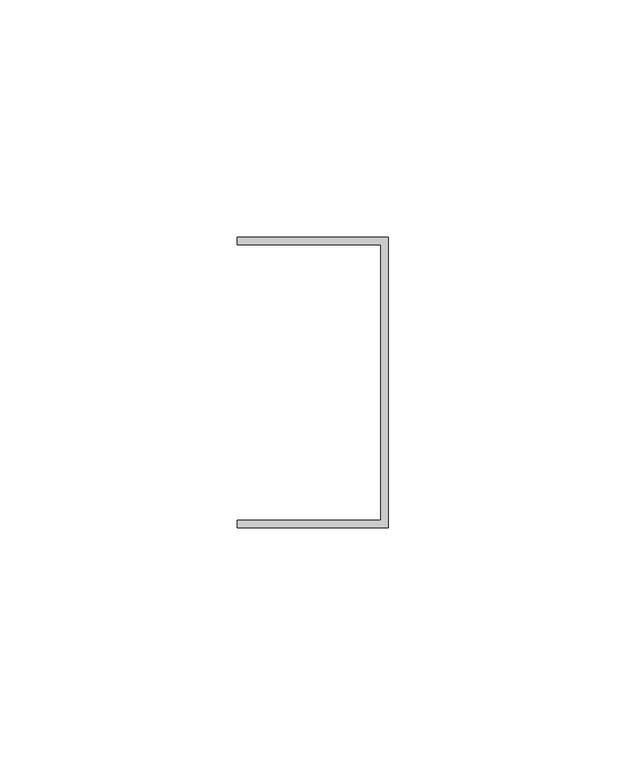
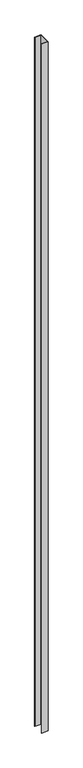
"""IFC4 building model written with IfcOpenShell, lengths in millimetres: proxy geometry, Generic Models 7:Generic Models 1:3:Generic Models 1:3 : Generic Models 7:Generic Models 1:305549:3:Generic Models 1:3:Generic Models 1:3 : Generic Models 7:Generic Models 1:305549:3 : Generic Models 7:Generic Models 1:3:Generic Models 1:3 : Generic Models 7:Generic Models 1:305549:301244:20 : Generic Models 7:Generic Models 1:3:Generic Models 1:3 : Generic Models 7:Generic Models 1:305549:3:Generic Models 1:3:Generic Models 1:3 : Generic Models 7:Generic Models 1:305549:3 : Generic Models 7:Generic Models 1:3:Generic Models 1:3 : Generic Models 7:Generic Models 1:305549:301244:308848."""

from ifc_helpers import new_model, si_unit, frame, origin, place, context, project, spatial, polyline, outline, extrude, source, transform, mapped, element, save


def generic_models_9a956034(model_context):
    return source(origin(), model_context, "Body", "SweptSolid", [
        extrude(outline(polyline([(594360.386724, -579015.772634), (594360.386724, -579076.8913841), (594328.636724, -579076.8913841), (594328.636724, -579075.3038841), (594358.799224, -579075.3038841), (594358.799224, -579017.360134), (594328.636724, -579017.360134), (594328.636724, -579015.772634), (594360.386724, -579015.772634)])), frame((0.0, 0.0, 50.8), z_axis=(0.0, 0.0, 1.0), x_axis=(1.0, 0.0, 0.0)), (0.0, 0.0, 1.0), 3657.6),
    ])


if __name__ == "__main__":
    model = new_model("IFC4")
    model_context = context("Model", 3, world=origin())
    ifc_project = project(units=[si_unit("LENGTHUNIT", "METRE", prefix="MILLI")], contexts=[model_context])
    site = spatial("IfcSite", under=ifc_project)
    building = spatial("IfcBuilding", under=site)
    placement = place(None, origin())
    generic_models_shape = generic_models_9a956034(model_context)
    element("IfcBuildingElementProxy", 1, Name="Generic Models 7:Generic Models 1:3:Generic Models 1:3 : Generic Models 7:Generic Models 1:305549:3:Generic Models 1:3:Generic Models 1:3 : Generic Models 7:Generic Models 1:305549:3 : Generic Models 7:Generic Models 1:3:Generic Models 1:3 : Generic Models 7:Generic Models 1:305549:301244:20 : Generic Models 7:Generic Models 1:3:Generic Models 1:3 : Generic Models 7:Generic Models 1:305549:3:Generic Models 1:3:Generic Models 1:3 : Generic Models 7:Generic Models 1:305549:3 : Generic Models 7:Generic Models 1:3:Generic Models 1:3 : Generic Models 7:Generic Models 1:305549:301244:308848", ObjectType="Generic Models 7:Generic Models 1:3:Generic Models 1:3 : Generic Models 7:Generic Models 1:305549:3:Generic Models 1:3:Generic Models 1:3 : Generic Models 7:Generic Models 1:305549:3 : Generic Models 7:Generic Models 1:3:Generic Models 1:3 : Generic Models 7:Generic Models 1:305549:301244:20 : Generic Models 7:Generic Models 1:3:Generic Models 1:3 : Generic Models 7:Generic Models 1:305549:3:Generic Models 1:3:Generic Models 1:3 : Generic Models 7:Generic Models 1:305549:3 : Generic Models 7:Generic Models 1:3:Generic Models 1:3 : Generic Models 7:Generic Models 1:305549:301244:308848", at=placement, inside=building, context=model_context, shape_type="MappedRepresentation", body=[
        mapped(generic_models_shape, transform((0.0, 0.0, 0.0), x_axis=(1.0, 0.0, 0.0), y_axis=(0.0, 1.0, 0.0), z_axis=(0.0, 0.0, 1.0))),
    ])
    save(model, "model.ifc")

# Revit data of these elements
# Type "Generic Models 7:Generic Models 1:3:Generic Models 1:3 : Generic Models 7:Generic Models 1:305549:3:Generic Models 1:3:Generic Models 1:3 : Generic Models 7:Generic Models 1:305549:3 : Generic Models 7:Generic Models 1:3:Generic Models 1:3 : Generic Models 7:Generic Models 1:305549:301244:20 : Generic Models 7:Generic Models 1:3:Generic Models 1:3 : Generic Models 7:Generic Models 1:305549:3:Generic Models 1:3:Generic Models 1:3 : Generic Models 7:Generic Models 1:305549:3 : Generic Models 7:Generic Models 1:3:Generic Models 1:3 : Generic Models 7:Generic Models 1:305549:301244:308848"
#   NameOverride = "Generic Models 7:Generic Models 1:3:Generic Models 1:3 : Generic Models 7:Generic Models 1:305549:3:Generic Models 1:3:Generic Models 1:3 : Generic Models 7:Generic Models 1:305549:3 : Generic Models 7:Generic Models 1:3:Generic Models 1:3 : Generic Models 7:Generic Models 1:305549:301244:308848"
#   ObjectTypeOverride = "Generic Models 1:3:Generic Models 1:3 : Generic Models 7:Generic Models 1:305549:3 : Generic Models 7:Generic Models 1:3:Generic Models 1:3 : Generic Models 7:Generic Models 1:305549:301244"
#   Reference = "Generic Models 1"
#   Tag = "308848"
# Element 1 (IfcBuildingElementProxy, "Generic Models 7:Generic Models 1:3:Generic Models 1:3 : Generic Models 7:Generic Models 1:305549:3:Generic Models 1:3:Generic Models 1:3 : Generic Models 7:Generic Models 1:305549:3 : Generic Models 7:Generic Models 1:3:Generic Models 1:3 : Generic Models 7:Generic Models 1:305549:301244:20 : Generic Models 7:Generic Models 1:3:Generic Models 1:3 : Generic Models 7:Generic Models 1:305549:3:Generic Models 1:3:Generic Models 1:3 : Generic Models 7:Generic Models 1:305549:3 : Generic Models 7:Generic Models 1:3:Generic Models 1:3 : Generic Models 7:Generic Models 1:305549:301244:308848")
#   Materials on its faces: "GALVANIZED U-CHANNEL (250T125-33)"
# Materials
#   "GALVANIZED U-CHANNEL (250T125-33)": class "Unassigned", colour RGB 202 201 200, transparency 0, Keynote = "M05451300.02", Cost = 0
